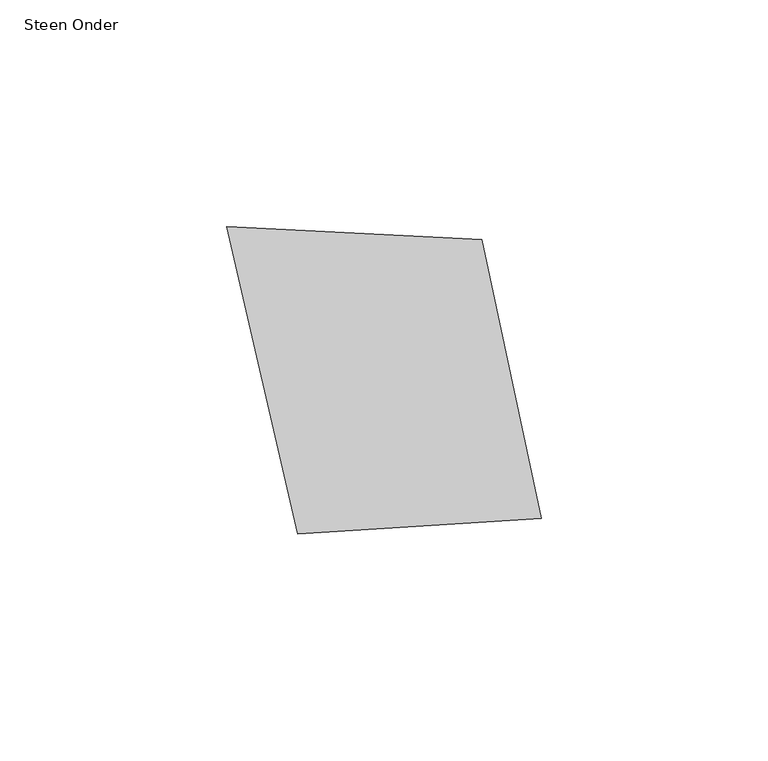
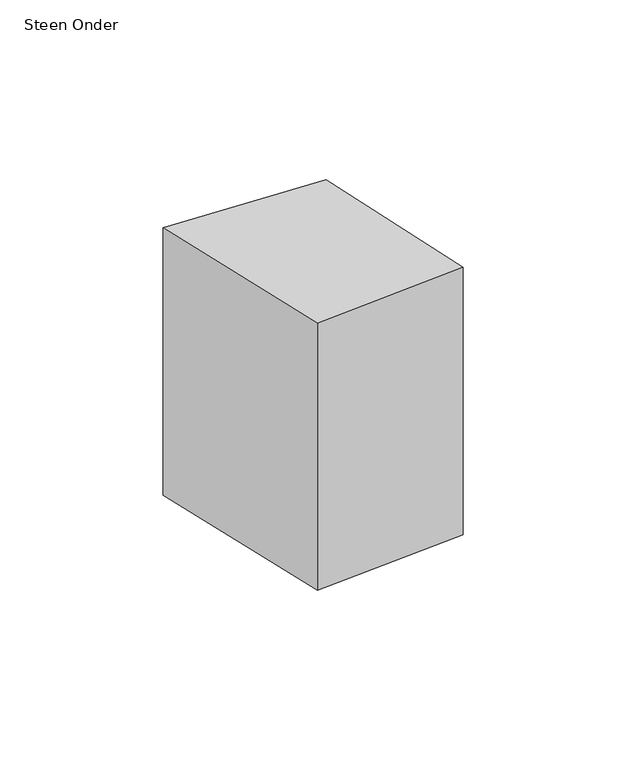
"""IFC4 building model written with IfcOpenShell, lengths in millimetres: proxy geometry, 00_GMA_steen_versie_4 : Steen Onder."""

from ifc_helpers import new_model, si_unit, origin, origin_with_axes, place, context, project, spatial, polyline, outline, extrude, source, transform, mapped, element, save


def steen_onder_9aa2fa60(model_context):
    return source(origin(), model_context, "Body", "SweptSolid", [
        extrude(outline(polyline([(94.5552851, 97.0098875), (107.5952828, 35.5694511), (53.9689209, 32.1485584), (38.4042692, 99.8235878), (94.5552851, 97.0098875)])), origin_with_axes(), (0.0, 0.0, 1.0), 100.0),
    ])


if __name__ == "__main__":
    model = new_model("IFC4")
    model_context = context("Model", 3, world=origin())
    ifc_project = project(units=[si_unit("LENGTHUNIT", "METRE", prefix="MILLI")], contexts=[model_context])
    site = spatial("IfcSite", under=ifc_project)
    building = spatial("IfcBuilding", under=site)
    placement = place(None, origin())
    steen_onder_shape = steen_onder_9aa2fa60(model_context)
    element("IfcBuildingElementProxy", 1, Name="00_GMA_steen_versie_4 : Steen Onder", ObjectType="00_GMA_steen_versie_4 : Steen Onder", at=placement, inside=building, context=model_context, shape_type="MappedRepresentation", body=[
        mapped(steen_onder_shape, transform((0.0, 0.0, 0.0), x_axis=(1.0, 0.0, 0.0), y_axis=(0.0, 1.0, 0.0), z_axis=(0.0, 0.0, 1.0))),
    ])
    save(model, "model.ifc")

# Revit data of these elements
# Type "00_GMA_steen_versie_4 : Steen Onder"
#   StootVoegHalfBoven [instance default] = 5 mm
#   StootVoegHalf [instance default] = 5 mm
#   StootVoegBreedteOnder = 10 mm
#   StootVoegBreedteBoven = 10 mm
#   Steendikte = 100 mm
#   LintVoegOnderHalf = 0 mm
#   LintVoegOnder = 0 mm
#   LintVoegBovenHalf = 5 mm
#   LintVoegBoven = 10 mm
#   materiaal = none
#   MateriaalVoeg = none
#   Default Elevation = 0
